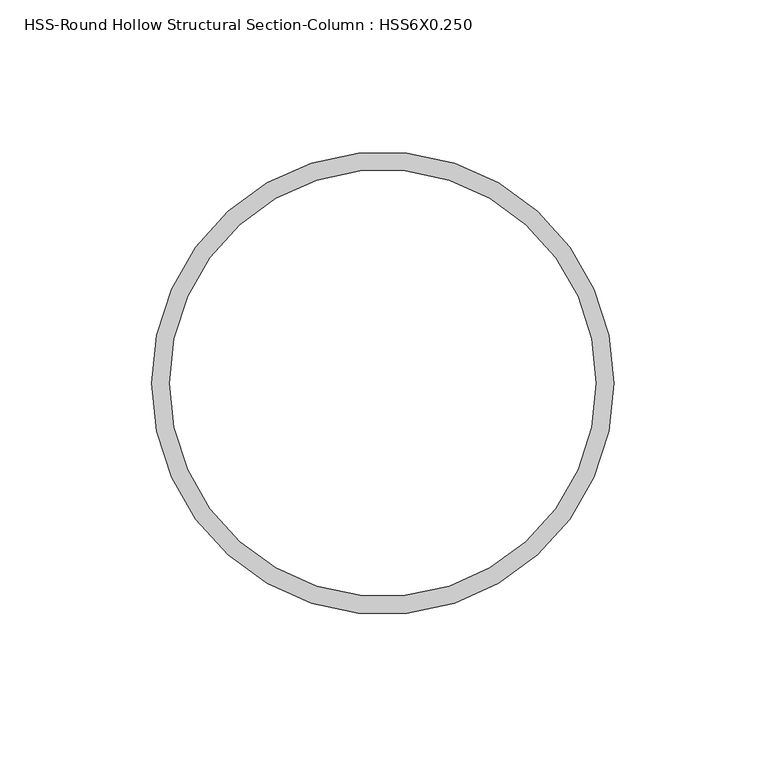
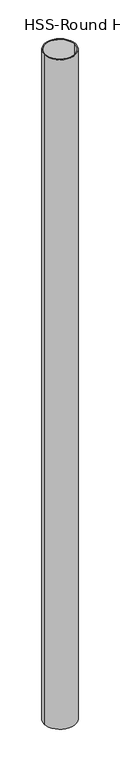
"""IFC4 building model written with IfcOpenShell, lengths in millimetres: column geometry, HSS-Round Hollow Structural Section-Column : HSS6X0.250."""

from ifc_helpers import new_model, si_unit, point, origin, origin_with_axes, origin_2d, place, context, project, spatial, circle_curve, trimmed, segment, composite_curve, outline, extrude, source, transform, mapped, element, save


def hss_round_hollow_structural_section_column_hss6x0_250_e49f8375(model_context):
    return source(origin(), model_context, "Body", "SweptSolid", [
        extrude(outline(composite_curve([segment(trimmed(circle_curve(origin_2d(), 76.2), [point((-76.2, 0.0))], [point((76.2, 0.0))], False, "CARTESIAN"), True, "CONTINUOUS"), segment(trimmed(circle_curve(origin_2d(), 76.2), [point((76.2, 0.0))], [point((-76.2, 0.0))], False, "CARTESIAN"), True, "CONTINUOUS")], self_intersect=False), holes=[composite_curve([segment(trimmed(circle_curve(origin_2d(), 70.2818), [point((-70.2818, 0.0))], [point((70.2818, 0.0))], True, "CARTESIAN"), True, "CONTINUOUS"), segment(trimmed(circle_curve(origin_2d(), 70.2818), [point((70.2818, 0.0))], [point((-70.2818, 0.0))], True, "CARTESIAN"), True, "CONTINUOUS")], self_intersect=False)]), origin_with_axes(), (0.0, 0.0, 1.0), 3403.6),
    ])


if __name__ == "__main__":
    model = new_model("IFC4")
    model_context = context("Model", 3, world=origin())
    ifc_project = project(units=[si_unit("LENGTHUNIT", "METRE", prefix="MILLI")], contexts=[model_context])
    site = spatial("IfcSite", under=ifc_project)
    building = spatial("IfcBuilding", under=site)
    placement = place(None, origin())
    hss_round_hollow_structural_section_column_hss6x0_250_shape = hss_round_hollow_structural_section_column_hss6x0_250_e49f8375(model_context)
    element("IfcColumn", 1, ObjectType="HSS-Round Hollow Structural Section-Column : HSS6X0.250", at=placement, inside=building, context=model_context, shape_type="MappedRepresentation", body=[
        mapped(hss_round_hollow_structural_section_column_hss6x0_250_shape, transform((0.0, 0.0, 0.0), x_axis=(1.0, 0.0, 0.0), y_axis=(0.0, 1.0, 0.0), z_axis=(0.0, 0.0, 1.0))),
    ])
    save(model, "model.ifc")

# Revit data of these elements
# Type "HSS-Round Hollow Structural Section-Column : HSS6X0.250"
#   Assembly Code = "B10"
#   W = 15.4
#   OD = 0' - 6"
#   t = 0' - 0.233"
#   A = 0.0293056 SF
#   Structural Material [instance default] = Steel ASTM A53
# Element 1 (IfcColumn, "HSS-Round Hollow Structural Section-Column : HSS6X0.250")
#   Materials on its faces: "Steel ASTM A53"
# Materials
#   "Steel ASTM A53": class "Metal", colour RGB 199 199 199, transparency 0, Description = "Carbon steel", Cost = 0
